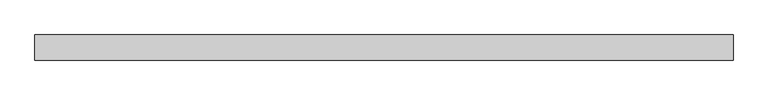
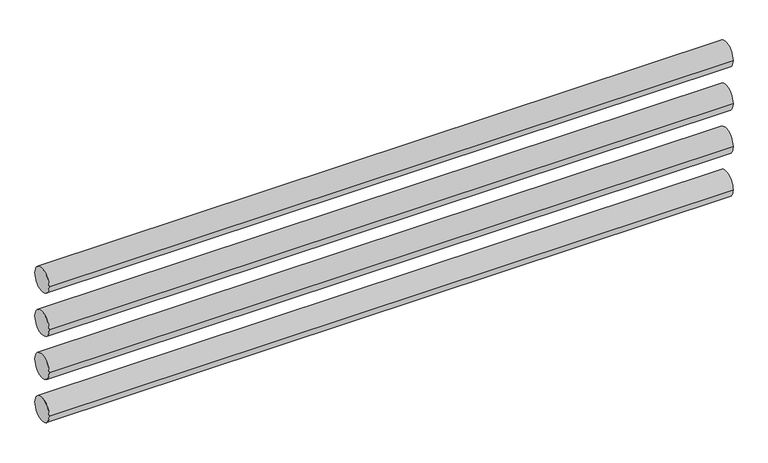
"""IFC4 building model written with IfcOpenShell, lengths in millimetres: proxy geometry, Газпремиум_Регистр : РГТ-1-108х3-3м-4."""

from ifc_helpers import new_model, si_unit, point, frame, frame_2d, origin, place, context, project, spatial, circle_curve, trimmed, segment, composite_curve, outline, extrude, source, transform, mapped, element, save


def mechanical_equipment_0300bfad(model_context):
    return source(origin(), model_context, "Body", "SweptSolid", [
        extrude(outline(composite_curve([segment(trimmed(circle_curve(frame_2d((0.0, 654.0)), 54.0), [point((-54.0, 654.0))], [point((54.0, 654.0))], False, "CARTESIAN"), True, "CONTINUOUS"), segment(trimmed(circle_curve(frame_2d((0.0, 654.0)), 54.0), [point((54.0, 654.0))], [point((-54.0, 654.0))], False, "CARTESIAN"), True, "CONTINUOUS")], self_intersect=False)), frame((-684.1719207, 0.0, 0.0), z_axis=(1.0, 0.0, 0.0), x_axis=(0.0, 1.0, 0.0)), (0.0, 0.0, 1.0), 3000.0),
        extrude(outline(composite_curve([segment(trimmed(circle_curve(frame_2d((0.0, 454.0)), 54.0), [point((-54.0, 454.0))], [point((54.0, 454.0))], False, "CARTESIAN"), True, "CONTINUOUS"), segment(trimmed(circle_curve(frame_2d((0.0, 454.0)), 54.0), [point((54.0, 454.0))], [point((-54.0, 454.0))], False, "CARTESIAN"), True, "CONTINUOUS")], self_intersect=False)), frame((-684.1719207, 0.0, 0.0), z_axis=(1.0, 0.0, 0.0), x_axis=(0.0, 1.0, 0.0)), (0.0, 0.0, 1.0), 3000.0),
        extrude(outline(composite_curve([segment(trimmed(circle_curve(frame_2d((0.0, 254.0)), 54.0), [point((-54.0, 254.0))], [point((54.0, 254.0))], False, "CARTESIAN"), True, "CONTINUOUS"), segment(trimmed(circle_curve(frame_2d((0.0, 254.0)), 54.0), [point((54.0, 254.0))], [point((-54.0, 254.0))], False, "CARTESIAN"), True, "CONTINUOUS")], self_intersect=False)), frame((-684.1719207, 0.0, 0.0), z_axis=(1.0, 0.0, 0.0), x_axis=(0.0, 1.0, 0.0)), (0.0, 0.0, 1.0), 3000.0),
        extrude(outline(composite_curve([segment(trimmed(circle_curve(frame_2d((0.0, 54.0)), 54.0), [point((-54.0, 54.0))], [point((54.0, 54.0))], False, "CARTESIAN"), True, "CONTINUOUS"), segment(trimmed(circle_curve(frame_2d((0.0, 54.0)), 54.0), [point((54.0, 54.0))], [point((-54.0, 54.0))], False, "CARTESIAN"), True, "CONTINUOUS")], self_intersect=False)), frame((-684.1719207, 0.0, 0.0), z_axis=(1.0, 0.0, 0.0), x_axis=(0.0, 1.0, 0.0)), (0.0, 0.0, 1.0), 3000.0),
    ])


if __name__ == "__main__":
    model = new_model("IFC4")
    model_context = context("Model", 3, world=origin())
    ifc_project = project(units=[si_unit("LENGTHUNIT", "METRE", prefix="MILLI")], contexts=[model_context])
    site = spatial("IfcSite", under=ifc_project)
    building = spatial("IfcBuilding", under=site)
    placement = place(None, origin())
    mechanical_equipment_shape = mechanical_equipment_0300bfad(model_context)
    element("IfcBuildingElementProxy", 1, Name="Газпремиум_Регистр : РГТ-1-108х3-3м-4", ObjectType="Газпремиум_Регистр : РГТ-1-108х3-3м-4", at=placement, inside=building, context=model_context, shape_type="MappedRepresentation", body=[
        mapped(mechanical_equipment_shape, transform((0.0, 0.0, 0.0), x_axis=(1.0, 0.0, 0.0), y_axis=(0.0, 1.0, 0.0), z_axis=(0.0, 0.0, 1.0))),
    ])
    save(model, "model.ifc")

# Revit data of these elements
# Type "Газпремиум_Регистр : РГТ-1-108х3-3м-4"
#   ADSK_Позиция = "390"
#   ADSK_Наименование = "Регистр однорядный из четырех гладких труб 108х3 длиной 3 м, в комплекте с опорами"
#   ADSK_Марка = "РГТ-1-108х3-3м-4-ОП-О ТУ 4936-001-69441315-11"
#   ADSK_Код изделия = "2050868"
#   ADSK_Завод-изготовитель = "ООО ПКП \"ГазПремиум\", Россия, г.Саратов, ИНН 6452951387, кпп 645201001, gaz-premium@mail.ru"
#   ADSK_Единица измерения = "шт."
#   Расстояние между рядами = 200 mm
#   Радиус.регистра = 54 mm
#   Отступ.труб.подкл.от.осевой = 32.719 mm
#   Длина регистра = 3000 mm
#   Диаметр.труб.подкл. = 32 mm
#   Диаметр регистра = 108 mm
#   Высота = 600 mm
#   ADSK_Масса = 141.71
#   ADSK_Количество = 1
#   Число рядов = 4
#   Соед.трубы = Грунтовка.красная
#   Регистр = Грунтовка.красная
#   Поддерж.арматура = Грунтовка.серая
#   Default Elevation = 0
# Element 1 (IfcBuildingElementProxy, "Газпремиум_Регистр : РГТ-1-108х3-3м-4")
#   Materials on its faces: "Грунтовка.красная"
# Materials
#   "Грунтовка.красная": class "Разное", colour RGB 255 0 0, transparency 0
#   "Грунтовка.серая": class "Разное", colour RGB 187 181 179, transparency 0
